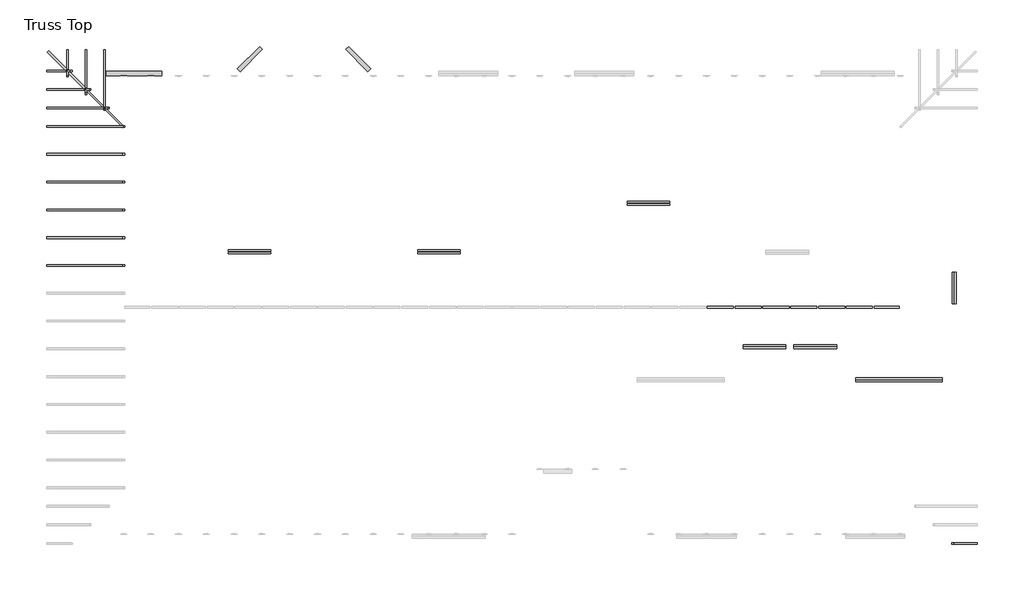
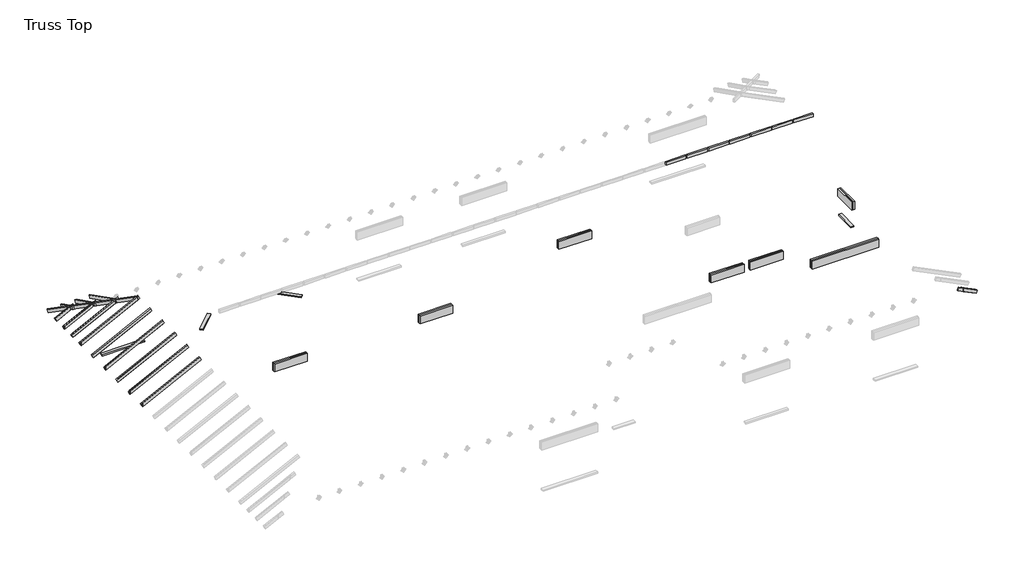
# One storey, part 2 of 3: 39 beams.
"""IFC4 building model written with IfcOpenShell, lengths in millimetres."""

import ifcopenshell
import ifcopenshell.guid

model = None  # the IFC model being written
_history = None  # IfcOwnerHistory: only IFC2X3 demands one
_inside = {}  # id of a spatial element -> (the spatial element, [elements in it])
_under = {}  # id of a project, library or spatial element -> (it, [spatial elements below it])
_declared = {}  # id of a project -> (the project, [libraries it declares])
_typed = {}  # id of a type object -> (the type object, [elements of that type])
_made_of = {}  # id of a material, layer set ... -> (it, [elements and type objects made of it])


def new_model(schema):
    """Start an empty IFC model of exactly this schema.

    Asked for "IFC4X3", IfcOpenShell would pick the latest addendum, in which some entities
    have other attributes; the version numbers below select the first issue.
    IFC2X3 requires an IfcOwnerHistory on every rooted entity: one is made here for all.
    """
    global model, _history
    if schema == "IFC4X3":
        model = ifcopenshell.file(schema_version=(4, 3, 0, 0))
    else:
        model = ifcopenshell.file(schema=schema)
    _inside.clear()
    _under.clear()
    _declared.clear()
    _typed.clear()
    _made_of.clear()
    _history = None
    if model.schema == "IFC2X3":
        org = make("IfcOrganization", Name="unknown")
        user = make(
            "IfcPersonAndOrganization",
            ThePerson=make("IfcPerson", FamilyName="unknown"),
            TheOrganization=org,
        )
        app = make(
            "IfcApplication",
            ApplicationDeveloper=org,
            Version="unknown",
            ApplicationFullName="unknown",
            ApplicationIdentifier="unknown",
        )
        _history = make(
            "IfcOwnerHistory",
            OwningUser=user,
            OwningApplication=app,
            ChangeAction="ADDED",
            CreationDate=0,
        )
    return model


def make(cls, **values):
    """One entity of the class cls with the attributes given. An attribute that is None is left unset."""
    return model.create_entity(
        cls, **{name: value for name, value in values.items() if value is not None}
    )


def rooted(cls, **values):
    """An entity with a GlobalId (a new one), such as an element, a storey or a relation."""
    return make(cls, GlobalId=ifcopenshell.guid.new(), OwnerHistory=_history, **values)


def si_unit(unit_type, name, prefix=None):
    """IfcSIUnit, for example si_unit("LENGTHUNIT", "METRE", prefix="MILLI")."""
    return make("IfcSIUnit", UnitType=unit_type, Prefix=prefix, Name=name)


def assignment(units):
    """IfcUnitAssignment: the units of a project."""
    return None if units is None else make("IfcUnitAssignment", Units=units)


def point(xyz):
    """IfcCartesianPoint."""
    return None if xyz is None else make("IfcCartesianPoint", Coordinates=xyz)


def direction(xyz):
    """IfcDirection."""
    return None if xyz is None else make("IfcDirection", DirectionRatios=xyz)


def frame(location, z_axis=None, x_axis=None):
    """IfcAxis2Placement3D, a coordinate frame: its origin and axes. An axis left out is left unset."""
    return make(
        "IfcAxis2Placement3D",
        Location=point(location),
        Axis=direction(z_axis),
        RefDirection=direction(x_axis),
    )


def origin():
    """The frame at (0, 0, 0) with its axes left unset."""
    return frame((0.0, 0.0, 0.0))


def place(relative_to, where):
    """IfcLocalPlacement: puts the frame where relative to a parent placement (None: the world)."""
    return make(
        "IfcLocalPlacement", PlacementRelTo=relative_to, RelativePlacement=where
    )


def context(
    kind, dimensions, precision=None, world=None, true_north=None, identifier=None
):
    """IfcGeometricRepresentationContext, for example the 3D "Model" context."""
    return make(
        "IfcGeometricRepresentationContext",
        ContextIdentifier=identifier,
        ContextType=kind,
        CoordinateSpaceDimension=dimensions,
        Precision=precision,
        WorldCoordinateSystem=world,
        TrueNorth=true_north,
    )


def project(units=None, contexts=None):
    """IfcProject with its units and contexts."""
    return rooted(
        "IfcProject",
        Name="project",
        RepresentationContexts=contexts,
        UnitsInContext=assignment(units),
    )


def spatial(cls, under=None, at=None, **own):
    """A site, building, storey or space (cls), placed at a placement, below another one or the project."""
    s = rooted(cls, ObjectPlacement=at, **own)
    if under is not None:
        _under.setdefault(under.id(), (under, []))[1].append(s)
    return s


def polyline(points):
    """IfcPolyline through the points."""
    return make("IfcPolyline", Points=[point(p) for p in points])


def outline(outer, holes=None, kind="AREA"):
    """IfcArbitraryClosedProfileDef: a profile drawn as a closed curve; with holes, ...WithVoids."""
    if holes is None:
        return make("IfcArbitraryClosedProfileDef", ProfileType=kind, OuterCurve=outer)
    return make(
        "IfcArbitraryProfileDefWithVoids",
        ProfileType=kind,
        OuterCurve=outer,
        InnerCurves=holes,
    )


def extrude(swept, where, along, depth):
    """IfcExtrudedAreaSolid: the profile swept, set in the frame where, extruded along a direction by depth."""
    return make(
        "IfcExtrudedAreaSolid",
        SweptArea=swept,
        Position=where,
        ExtrudedDirection=direction(along),
        Depth=depth,
    )


def faces_of(points, faces, orient=None, outer=None):
    """IfcFace entities. A face is a list of loops; a loop is a list of indices into points, from 0.

    orient and outer hold one flag for each loop. By default every Orientation is true, the
    first loop of a face is its IfcFaceOuterBound and the others are IfcFaceBound.
    """
    made = []
    for i, loops in enumerate(faces):
        bounds = []
        for j, loop in enumerate(loops):
            is_outer = j == 0 if outer is None else outer[i][j]
            bounds.append(
                make(
                    "IfcFaceOuterBound" if is_outer else "IfcFaceBound",
                    Bound=make("IfcPolyLoop", Polygon=[points[k] for k in loop]),
                    Orientation=True if orient is None else orient[i][j],
                )
            )
        made.append(make("IfcFace", Bounds=bounds))
    return made


def faceted_brep(points, faces, orient=None, outer=None, voids=None):
    """IfcFacetedBrep: a solid bounded by flat faces; with voids (closed shells), ...WithVoids."""
    shared = [point(p) for p in points]
    hull = make("IfcClosedShell", CfsFaces=faces_of(shared, faces, orient, outer))
    if voids is None:
        return make("IfcFacetedBrep", Outer=hull)
    return make(
        "IfcFacetedBrepWithVoids",
        Outer=hull,
        Voids=[
            make(cls, CfsFaces=faces_of(shared, fs, o, b)) for cls, fs, o, b in voids
        ],
    )


def shape(context_of_items, identifier, shape_type, items):
    """IfcShapeRepresentation: the items that make up one representation, for example the "Body"."""
    return make(
        "IfcShapeRepresentation",
        ContextOfItems=context_of_items,
        RepresentationIdentifier=identifier,
        RepresentationType=shape_type,
        Items=items,
    )


def source(mapping_origin, context_of_items, identifier, shape_type, items):
    """IfcRepresentationMap: a shape defined once, which mapped items show again and again."""
    return make(
        "IfcRepresentationMap",
        MappingOrigin=mapping_origin,
        MappedRepresentation=shape(context_of_items, identifier, shape_type, items),
    )


def transform(
    local_origin,
    x_axis=None,
    y_axis=None,
    z_axis=None,
    scale=None,
    scale2=None,
    scale3=None,
    uniform=True,
):
    """IfcCartesianTransformationOperator3D, or its non-uniform kind. x_axis, y_axis, z_axis: its Axis1, 2, 3."""
    if uniform:
        return make(
            "IfcCartesianTransformationOperator3D",
            Axis1=direction(x_axis),
            Axis2=direction(y_axis),
            LocalOrigin=point(local_origin),
            Scale=scale,
            Axis3=direction(z_axis),
        )
    return make(
        "IfcCartesianTransformationOperator3DnonUniform",
        Axis1=direction(x_axis),
        Axis2=direction(y_axis),
        LocalOrigin=point(local_origin),
        Scale=scale,
        Axis3=direction(z_axis),
        Scale2=scale2,
        Scale3=scale3,
    )


def mapped(mapping_source, mapping_target):
    """IfcMappedItem: shows the shape of a source again, moved by a transform."""
    return make(
        "IfcMappedItem", MappingSource=mapping_source, MappingTarget=mapping_target
    )


def made_of(thing, what):
    """Note that an element or type object is made of a material, layer set ...; save() writes the relation."""
    if what is not None:
        _made_of.setdefault(what.id(), (what, []))[1].append(thing)
    return thing


def element(
    cls,
    number,
    at=None,
    inside=None,
    cuts=None,
    type_object=None,
    material=None,
    context=None,
    identifier="Body",
    shape_type=None,
    held_by="IfcProductDefinitionShape",
    body=None,
    shapes=None,
    **own,
):
    """One element of the class cls, such as IfcWall. Its Tag is "e" and its number.

    at: its placement. inside: the storey or other place that contains it. cuts: it is an
    opening in that element (IfcRelVoidsElement). A single representation is given by context,
    identifier, shape_type and body (its items); several are given by shapes. held_by: the class
    of the entity that holds the representations. save() writes the other relations.
    """
    e = rooted(cls, Tag="e%d" % number, ObjectPlacement=at, **own)
    if body is not None:
        shapes = [shape(context, identifier, shape_type, body)]
    if shapes is not None:
        e.Representation = make(held_by, Representations=shapes)
    if inside is not None:
        _inside.setdefault(inside.id(), (inside, []))[1].append(e)
    if cuts is not None:
        rooted(
            "IfcRelVoidsElement", RelatingBuildingElement=cuts, RelatedOpeningElement=e
        )
    if type_object is not None:
        _typed.setdefault(type_object.id(), (type_object, []))[1].append(e)
    return made_of(e, material)


def aggregate(whole, parts):
    """IfcRelAggregates: a whole, such as a stair, and the parts it consists of."""
    return rooted("IfcRelAggregates", RelatingObject=whole, RelatedObjects=parts)


def save(model, path):
    """Write the relations noted so far, then the file.

    IfcRelAggregates (storeys below a building ...), IfcRelContainedInSpatialStructure (elements
    in a storey), IfcRelDefinesByType, IfcRelAssociatesMaterial and IfcRelDeclares: one each for
    every whole, place, type object, material and project.
    """
    for whole, parts in _under.values():
        aggregate(whole, parts)
    for where, things in _inside.values():
        rooted(
            "IfcRelContainedInSpatialStructure",
            RelatedElements=things,
            RelatingStructure=where,
        )
    for kind, things in _typed.values():
        rooted("IfcRelDefinesByType", RelatedObjects=things, RelatingType=kind)
    for what, things in _made_of.values():
        rooted("IfcRelAssociatesMaterial", RelatedObjects=things, RelatingMaterial=what)
    for by, libraries in _declared.values():
        rooted("IfcRelDeclares", RelatingContext=by, RelatedDefinitions=libraries)
    model.write(path)


def dimension_lumber_02b3d2e5(model_context):
    return source(origin(), model_context, "Body", "SweptSolid", [
        extrude(outline(polyline([(1211.111892, 19.05), (1211.111892, -19.05), (-1244.9189714, -19.05), (-1244.9189714, 19.05), (1211.111892, 19.05)])), frame((0.0, 0.0, -44.45), z_axis=(0.0, 0.0, 1.0), x_axis=(1.0, 0.0, 0.0)), (0.0, 0.0, 1.0), 88.9),
    ])


def dimension_lumber_26660400(model_context):
    return source(origin(), model_context, "Body", "SweptSolid", [
        extrude(outline(polyline([(276.225, 19.05), (276.225, -19.05), (-276.225, -19.05), (-276.225, 19.05), (276.225, 19.05)])), frame((0.0, 0.0, -44.45), z_axis=(0.0, 0.0, 1.0), x_axis=(1.0, 0.0, 0.0)), (0.0, 0.0, 1.0), 88.9),
    ])


def dimension_lumber_d546034e(model_context):
    return source(origin(), model_context, "Body", "SweptSolid", [
        extrude(outline(polyline([(295.275, 19.05), (295.275, -19.05), (-276.225, -19.05), (-276.225, 19.05), (295.275, 19.05)])), frame((0.0, 0.0, -44.45), z_axis=(0.0, 0.0, 1.0), x_axis=(1.0, 0.0, 0.0)), (0.0, 0.0, 1.0), 88.9),
    ])


def dimension_lumber_37c2d9e3(model_context):
    return source(origin(), model_context, "Body", "SweptSolid", [
        extrude(outline(polyline([(609.5999994, 44.45), (609.5999994, -44.45), (-609.5999994, -44.45), (-609.5999994, 44.45), (609.5999994, 44.45)])), frame((0.0, 0.0, -19.05), z_axis=(0.0, 0.0, 1.0), x_axis=(1.0, 0.0, 0.0)), (0.0, 0.0, 1.0), 38.1),
    ])


def dimension_lumber_e295fb9e(model_context):
    return source(origin(), model_context, "Body", "SweptSolid", [
        extrude(outline(polyline([(333.375, 44.45), (333.375, -44.45), (-352.4249994, -44.45), (-352.4249994, 44.45), (333.375, 44.45)])), frame((0.0, 0.0, -19.05), z_axis=(0.0, 0.0, 1.0), x_axis=(1.0, 0.0, 0.0)), (0.0, 0.0, 1.0), 38.1),
    ])


def dimension_lumber_05c0664a(model_context):
    return source(origin(), model_context, "Body", "SweptSolid", [
        extrude(outline(polyline([(333.375, -44.45), (-352.4249994, -44.45), (-352.4249994, 44.45), (333.375, 44.45), (333.375, -44.45)])), frame((0.0, 0.0, -19.05), z_axis=(0.0, 0.0, 1.0), x_axis=(1.0, 0.0, 0.0)), (0.0, 0.0, 1.0), 38.1),
    ])


def dimension_lumber_0879c48f(model_context):
    return source(origin(), model_context, "Body", "SweptSolid", [
        extrude(outline(polyline([(304.8, 44.45), (304.8, -44.45), (-304.8, -44.45), (-304.8, 44.45), (304.8, 44.45)])), frame((0.0, 0.0, -19.05), z_axis=(0.0, 0.0, 1.0), x_axis=(1.0, 0.0, 0.0)), (0.0, 0.0, 1.0), 38.1),
    ])


def dimension_lumber_2x10_header_exterior_80556d04(model_context):
    return source(origin(), model_context, "Body", "SweptSolid", [
        extrude(outline(polyline([(265.509375, 19.05), (265.509375, -19.05), (-420.290625, -19.05), (-420.290625, 19.05), (265.509375, 19.05)])), frame((0.0, 0.0, -117.475), z_axis=(0.0, 0.0, 1.0), x_axis=(1.0, 0.0, 0.0)), (0.0, 0.0, 1.0), 234.95),
    ])


def dimension_lumber_2x10_header_exterior_dd7e88d1(model_context):
    return source(origin(), model_context, "Body", "SweptSolid", [
        extrude(outline(polyline([(468.709375, 19.05), (468.709375, -19.05), (-468.709375, -19.05), (-468.709375, 19.05), (468.709375, 19.05)])), frame((0.0, 0.0, -117.475), z_axis=(0.0, 0.0, 1.0), x_axis=(1.0, 0.0, 0.0)), (0.0, 0.0, 1.0), 234.95),
    ])


def dimension_lumber_2x10_header_interior_e412fa49(model_context):
    return source(origin(), model_context, "Body", "SweptSolid", [
        extrude(outline(polyline([(468.709375, 19.05), (468.709375, -19.05), (-471.090625, -19.05), (-471.090625, 19.05), (468.709375, 19.05)])), frame((0.0, 0.0, -117.475), z_axis=(0.0, 0.0, 1.0), x_axis=(1.0, 0.0, 0.0)), (0.0, 0.0, 1.0), 234.95),
    ])


def dimension_lumber_2x10_header_interior_91014728(model_context):
    return source(origin(), model_context, "Body", "SweptSolid", [
        extrude(outline(polyline([(468.709375, 19.05), (468.709375, -19.05), (-1434.7031244, -19.05), (-1434.7031244, 19.05), (468.709375, 19.05)])), frame((0.0, 0.0, -117.475), z_axis=(0.0, 0.0, 1.0), x_axis=(1.0, 0.0, 0.0)), (0.0, 0.0, 1.0), 234.95),
    ])


model = new_model("IFC4")

# Units and contexts
model_context = context("Model", 3, world=origin())
ifc_project = project(units=[si_unit("LENGTHUNIT", "METRE", prefix="MILLI")], contexts=[model_context])

# Site, building, storey
site = spatial("IfcSite", under=ifc_project)
building = spatial("IfcBuilding", under=site)
storey = spatial("IfcBuildingStorey", under=building, Name="Truss Top", Elevation=5452.4432216)

# Beams
placement = place(None, origin())
element("IfcBeam", 1, ObjectType="Dimension Lumber : Roof Lumbers", at=placement, inside=storey, context=model_context, shape_type="SweptSolid", body=[
    extrude(outline(polyline([(0.0, -38.1), (0.0, 0.0), (1874.2721787, 0.0), (1874.2721787, -38.1), (0.0, -38.1)])), frame((-6669.4579365, 251.1959053, 2554.840297), z_axis=(-0.44721359549993395, 0.0, 0.894427190999928), x_axis=(0.894427190999928, 0.0, 0.44721359549993395)), (0.0, 0.0, 1.0), 88.9),
    extrude(outline(polyline([(2558.1548743, -6671.1152251), (2554.840297, -6669.4579365), (3393.040297, -4993.0579365), (3472.5548743, -5032.8152251), (2653.4048743, -6671.1152251), (2558.1548743, -6671.1152251)])), frame((0.0, 213.0959053, 0.0), z_axis=(0.0, 1.0, 0.0), x_axis=(0.0, 0.0, 1.0)), (0.0, 0.0, 1.0), 38.1),
    extrude(outline(polyline([(2564.60625, -6649.9260305), (3393.040297, -4993.0579365), (3472.5548743, -5032.8152251), (2653.4048743, -6671.1152251), (2564.60625, -6671.1152251), (2564.60625, -6649.9260305)])), frame((0.0, 213.0959053, 0.0), z_axis=(0.0, 1.0, 0.0), x_axis=(0.0, 0.0, 1.0)), (0.0, 0.0, 1.0), 38.1),
    extrude(outline(polyline([(2564.60625, -6649.9260305), (3373.1616527, -5032.8152251), (3472.5548743, -5032.8152251), (2653.4048743, -6671.1152251), (2564.60625, -6671.1152251), (2564.60625, -6649.9260305)])), frame((0.0, 213.0959053, 0.0), z_axis=(0.0, 1.0, 0.0), x_axis=(0.0, 0.0, 1.0)), (0.0, 0.0, 1.0), 38.1),
])
element("IfcBeam", 2, ObjectType="Dimension Lumber : Roof Lumbers", at=placement, inside=storey, context=model_context, shape_type="SweptSolid", body=[
    extrude(outline(polyline([(0.0, -38.1), (0.0, 0.0), (1874.2721787, 0.0), (1874.2721787, -38.1), (0.0, -38.1)])), frame((-6669.4579365, 860.7959053, 2554.840297), z_axis=(-0.44721359549993367, 0.0, 0.8944271909999281), x_axis=(0.8944271909999281, 0.0, 0.44721359549993367)), (0.0, 0.0, 1.0), 88.9),
    extrude(outline(polyline([(2558.1548743, -6671.1152251), (2554.840297, -6669.4579365), (3393.040297, -4993.0579365), (3472.5548743, -5032.8152251), (2653.4048743, -6671.1152251), (2558.1548743, -6671.1152251)])), frame((0.0, 822.6959053, 0.0), z_axis=(0.0, 1.0, 0.0), x_axis=(0.0, 0.0, 1.0)), (0.0, 0.0, 1.0), 38.1),
    extrude(outline(polyline([(2564.60625, -6649.9260305), (3393.040297, -4993.0579365), (3472.5548743, -5032.8152251), (2653.4048743, -6671.1152251), (2564.60625, -6671.1152251), (2564.60625, -6649.9260305)])), frame((0.0, 822.6959053, 0.0), z_axis=(0.0, 1.0, 0.0), x_axis=(0.0, 0.0, 1.0)), (0.0, 0.0, 1.0), 38.1),
    extrude(outline(polyline([(2564.60625, -6649.9260305), (3373.1616527, -5032.8152251), (3472.5548743, -5032.8152251), (2653.4048743, -6671.1152251), (2564.60625, -6671.1152251), (2564.60625, -6649.9260305)])), frame((0.0, 822.6959053, 0.0), z_axis=(0.0, 1.0, 0.0), x_axis=(0.0, 0.0, 1.0)), (0.0, 0.0, 1.0), 38.1),
])
element("IfcBeam", 3, ObjectType="Dimension Lumber : Roof Lumbers", at=placement, inside=storey, context=model_context, shape_type="SweptSolid", body=[
    extrude(outline(polyline([(0.0, -38.1), (0.0, 0.0), (1874.2721787, 0.0), (1874.2721787, -38.1), (0.0, -38.1)])), frame((-6669.4579365, 1470.3959053, 2554.840297), z_axis=(-0.44721359549993367, 0.0, 0.8944271909999281), x_axis=(0.8944271909999281, 0.0, 0.44721359549993367)), (0.0, 0.0, 1.0), 88.9),
    extrude(outline(polyline([(2558.1548743, -6671.1152251), (2554.840297, -6669.4579365), (3393.040297, -4993.0579365), (3472.5548743, -5032.8152251), (2653.4048743, -6671.1152251), (2558.1548743, -6671.1152251)])), frame((0.0, 1432.2959053, 0.0), z_axis=(0.0, 1.0, 0.0), x_axis=(0.0, 0.0, 1.0)), (0.0, 0.0, 1.0), 38.1),
    extrude(outline(polyline([(2564.60625, -6649.9260305), (3393.040297, -4993.0579365), (3472.5548743, -5032.8152251), (2653.4048743, -6671.1152251), (2564.60625, -6671.1152251), (2564.60625, -6649.9260305)])), frame((0.0, 1432.2959053, 0.0), z_axis=(0.0, 1.0, 0.0), x_axis=(0.0, 0.0, 1.0)), (0.0, 0.0, 1.0), 38.1),
    extrude(outline(polyline([(2564.60625, -6649.9260305), (3373.1616527, -5032.8152251), (3472.5548743, -5032.8152251), (2653.4048743, -6671.1152251), (2564.60625, -6671.1152251), (2564.60625, -6649.9260305)])), frame((0.0, 1432.2959053, 0.0), z_axis=(0.0, 1.0, 0.0), x_axis=(0.0, 0.0, 1.0)), (0.0, 0.0, 1.0), 38.1),
])
element("IfcBeam", 4, ObjectType="Dimension Lumber : Roof Lumbers", at=placement, inside=storey, context=model_context, shape_type="SweptSolid", body=[
    extrude(outline(polyline([(0.0, -38.1), (0.0, 0.0), (1874.2721787, 0.0), (1874.2721787, -38.1), (0.0, -38.1)])), frame((-6669.4579365, 2079.9959053, 2554.840297), z_axis=(-0.4472135954999335, 0.0, 0.8944271909999282), x_axis=(0.8944271909999282, 0.0, 0.4472135954999335)), (0.0, 0.0, 1.0), 88.9),
    extrude(outline(polyline([(2558.1548743, -6671.1152251), (2554.840297, -6669.4579365), (3393.040297, -4993.0579365), (3472.5548743, -5032.8152251), (2653.4048743, -6671.1152251), (2558.1548743, -6671.1152251)])), frame((0.0, 2041.8959053, 0.0), z_axis=(0.0, 1.0, 0.0), x_axis=(0.0, 0.0, 1.0)), (0.0, 0.0, 1.0), 38.1),
    extrude(outline(polyline([(2564.60625, -6649.9260305), (3393.040297, -4993.0579365), (3472.5548743, -5032.8152251), (2653.4048743, -6671.1152251), (2564.60625, -6671.1152251), (2564.60625, -6649.9260305)])), frame((0.0, 2041.8959053, 0.0), z_axis=(0.0, 1.0, 0.0), x_axis=(0.0, 0.0, 1.0)), (0.0, 0.0, 1.0), 38.1),
    extrude(outline(polyline([(2564.60625, -6649.9260305), (3373.1616527, -5032.8152251), (3472.5548743, -5032.8152251), (2653.4048743, -6671.1152251), (2564.60625, -6671.1152251), (2564.60625, -6649.9260305)])), frame((0.0, 2041.8959053, 0.0), z_axis=(0.0, 1.0, 0.0), x_axis=(0.0, 0.0, 1.0)), (0.0, 0.0, 1.0), 38.1),
])
element("IfcBeam", 5, ObjectType="Dimension Lumber : Roof Lumbers", at=placement, inside=storey, context=model_context, shape_type="SweptSolid", body=[
    extrude(outline(polyline([(0.0, -38.1), (0.0, 0.0), (1874.2721787, 0.0), (1874.2721787, -38.1), (0.0, -38.1)])), frame((-6669.4579365, 2689.5959053, 2554.840297), z_axis=(-0.4472135954999337, 0.0, 0.8944271909999281), x_axis=(0.8944271909999281, 0.0, 0.4472135954999337)), (0.0, 0.0, 1.0), 88.9),
    extrude(outline(polyline([(2558.1548743, -6671.1152251), (2554.840297, -6669.4579365), (3393.040297, -4993.0579365), (3472.5548743, -5032.8152251), (2653.4048743, -6671.1152251), (2558.1548743, -6671.1152251)])), frame((0.0, 2651.4959053, 0.0), z_axis=(0.0, 1.0, 0.0), x_axis=(0.0, 0.0, 1.0)), (0.0, 0.0, 1.0), 38.1),
    extrude(outline(polyline([(2564.60625, -6649.9260305), (3393.040297, -4993.0579365), (3472.5548743, -5032.8152251), (2653.4048743, -6671.1152251), (2564.60625, -6671.1152251), (2564.60625, -6649.9260305)])), frame((0.0, 2651.4959053, 0.0), z_axis=(0.0, 1.0, 0.0), x_axis=(0.0, 0.0, 1.0)), (0.0, 0.0, 1.0), 38.1),
    extrude(outline(polyline([(2564.60625, -6649.9260305), (3373.1616527, -5032.8152251), (3472.5548743, -5032.8152251), (2653.4048743, -6671.1152251), (2564.60625, -6671.1152251), (2564.60625, -6649.9260305)])), frame((0.0, 2651.4959053, 0.0), z_axis=(0.0, 1.0, 0.0), x_axis=(0.0, 0.0, 1.0)), (0.0, 0.0, 1.0), 38.1),
])
element("IfcBeam", 6, ObjectType="Dimension Lumber : Roof Lumbers", at=placement, inside=storey, context=model_context, shape_type="SweptSolid", body=[
    extrude(outline(polyline([(0.0, 38.1), (1877.0701871, 38.1), (1877.0701871, 0.0), (0.0, 0.0), (0.0, 38.1)])), frame((-6669.4579365, 3261.0959053, 2554.840297), z_axis=(-0.44721359549993367, 0.0, 0.8944271909999281), x_axis=(0.8944271909999281, 0.0, 0.44721359549993367)), (0.0, 0.0, 1.0), 88.9),
    extrude(outline(polyline([(2554.840297, -6669.4579365), (3394.2916044, -4990.5553218), (3473.8061816, -5030.3126104), (2653.4048743, -6671.1152251), (2558.1548743, -6671.1152251), (2554.840297, -6669.4579365)])), frame((0.0, 3261.0959053, 0.0), z_axis=(0.0, 1.0, 0.0), x_axis=(0.0, 0.0, 1.0)), (0.0, 0.0, 1.0), 38.1),
    extrude(outline(polyline([(2564.60625, -6649.9260305), (3394.2916044, -4990.5553218), (3473.8061816, -5030.3126104), (2653.4048743, -6671.1152251), (2564.60625, -6671.1152251), (2564.60625, -6649.9260305)])), frame((0.0, 3261.0959053, 0.0), z_axis=(0.0, 1.0, 0.0), x_axis=(0.0, 0.0, 1.0)), (0.0, 0.0, 1.0), 38.1),
    extrude(outline(polyline([(2564.60625, -6649.9260305), (3373.1616527, -5032.8152251), (3472.5548743, -5032.8152251), (2653.4048743, -6671.1152251), (2564.60625, -6671.1152251), (2564.60625, -6649.9260305)])), frame((0.0, 3261.0959053, 0.0), z_axis=(0.0, 1.0, 0.0), x_axis=(0.0, 0.0, 1.0)), (0.0, 0.0, 1.0), 38.1),
])
element("IfcBeam", 7, ObjectType="Dimension Lumber : Roof Lumbers", at=placement, inside=storey, context=model_context, shape_type="Brep", body=[
    faceted_brep([(13712.3847749, -5882.9040947, 2634.3548743), (13672.6274862, -5882.9040947, 2554.840297), (13672.6274862, -5844.8040947, 2554.840297), (13712.3847749, -5844.8040947, 2634.3548743), (13189.8604099, -5882.9040947, 2895.6170568), (13189.8604099, -5844.8040947, 2895.6170568), (13150.1031213, -5844.8040947, 2816.1024795), (13150.1031213, -5882.9040947, 2816.1024795)], [[[0, 1, 2, 3]], [[4, 5, 6, 7]], [[3, 5, 4, 0]], [[2, 6, 5, 3]], [[1, 7, 6, 2]], [[0, 4, 7, 1]]]),
    faceted_brep([(13712.3847749, -5882.9040947, 2634.3548743), (13672.6274862, -5882.9040947, 2554.840297), (13672.6274862, -5844.8040947, 2554.840297), (13712.3847749, -5844.8040947, 2634.3548743), (13301.1755432, -5882.9040947, 2839.9594901), (13301.1755432, -5882.9040947, 2740.5662685), (13263.0755432, -5844.8040947, 2759.6162685), (13263.0755432, -5844.8040947, 2859.0094901)], [[[0, 1, 2, 3]], [[0, 4, 5, 1]], [[1, 5, 6, 2]], [[2, 6, 7, 3]], [[3, 7, 4, 0]], [[4, 7, 6, 5]]]),
    faceted_brep([(13674.2847749, -5882.9040947, 2558.1548743), (13674.2847749, -5844.8040947, 2558.1548743), (13674.2847749, -5844.8040947, 2653.4048743), (13674.2847749, -5882.9040947, 2653.4048743), (13672.6274862, -5882.9040947, 2554.840297), (13672.6274862, -5844.8040947, 2554.840297), (13301.1755432, -5882.9040947, 2839.9594901), (13301.1755432, -5882.9040947, 2740.5662685), (13263.0755432, -5844.8040947, 2759.6162685), (13263.0755432, -5844.8040947, 2859.0094901)], [[[0, 1, 2, 3]], [[0, 4, 5, 1]], [[3, 6, 7, 4, 0]], [[4, 7, 8, 5]], [[5, 8, 9, 2, 1]], [[2, 9, 6, 3]], [[6, 9, 8, 7]]]),
])
element("IfcBeam", 8, ObjectType="Dimension Lumber : Roof Lumbers", at=placement, inside=storey, context=model_context, shape_type="Brep", body=[
    faceted_brep([(-5458.2652251, 3677.4390525, 3273.9083007), (-5458.2652251, 3637.6817638, 3194.3937234), (-5420.1652251, 3637.6817638, 3194.3937234), (-5420.1652251, 3677.4390525, 3273.9083007), (-5458.2652251, 4964.5299027, 2630.3628756), (-5420.1652251, 4964.5299027, 2630.3628756), (-5420.1652251, 4924.7726141, 2550.8482983), (-5458.2652251, 4924.7726141, 2550.8482983)], [[[0, 1, 2, 3]], [[4, 5, 6, 7]], [[3, 5, 4, 0]], [[2, 6, 5, 3]], [[1, 7, 6, 2]], [[0, 4, 7, 1]]]),
    faceted_brep([(-5458.2652251, 4964.5299027, 2630.3628756), (-5420.1652251, 4964.5299027, 2630.3628756), (-5420.1652251, 4924.7726141, 2550.8482983), (-5458.2652251, 4924.7726141, 2550.8482983), (-5420.1652251, 3694.4366737, 3265.4094901), (-5458.2652251, 3732.5366737, 3246.3594901), (-5420.1652251, 3694.4366737, 3166.0162685), (-5458.2652251, 3732.5366737, 3146.9662685)], [[[0, 1, 2, 3]], [[4, 1, 0, 5]], [[6, 2, 1, 4]], [[7, 3, 2, 6]], [[5, 0, 3, 7]], [[4, 5, 7, 6]]]),
    faceted_brep([(-5420.1652251, 3694.4366737, 3166.0162685), (-5420.1652251, 4918.4459053, 2554.0116527), (-5420.1652251, 4918.4459053, 2653.4048743), (-5420.1652251, 3694.4366737, 3265.4094901), (-5458.2652251, 4918.4459053, 2653.4048743), (-5458.2652251, 3732.5366737, 3246.3594901), (-5458.2652251, 4918.4459053, 2554.0116527), (-5458.2652251, 3732.5366737, 3146.9662685)], [[[0, 1, 2, 3]], [[3, 2, 4, 5]], [[5, 4, 6, 7]], [[3, 5, 7, 0]], [[7, 6, 1, 0]], [[4, 2, 1, 6]]]),
    faceted_brep([(-5458.2652251, 3732.5366737, 3146.9662685), (-5458.2652251, 4897.2567107, 2564.60625), (-5420.1652251, 4897.2567107, 2564.60625), (-5420.1652251, 3694.4366737, 3166.0162685), (-5420.1652251, 4918.4459053, 2564.60625), (-5420.1652251, 4918.4459053, 2653.4048743), (-5420.1652251, 3694.4366737, 3265.4094901), (-5458.2652251, 4918.4459053, 2653.4048743), (-5458.2652251, 4918.4459053, 2564.60625), (-5458.2652251, 3732.5366737, 3246.3594901)], [[[0, 1, 2, 3]], [[3, 2, 4, 5, 6]], [[7, 5, 4, 8]], [[6, 5, 7, 9]], [[6, 9, 0, 3]], [[9, 7, 8, 1, 0]], [[4, 2, 1, 8]]]),
])
element("IfcBeam", 9, ObjectType="Dimension Lumber : Roof Lumbers", at=placement, inside=storey, context=model_context, shape_type="Brep", body=[
    faceted_brep([(-5864.6652251, 4020.6444286, 3102.3056127), (-5864.6652251, 3980.88714, 3022.7910354), (-5826.5652251, 3980.88714, 3022.7910354), (-5826.5652251, 4020.6444286, 3102.3056127), (-5864.6652251, 4964.5299027, 2630.3628756), (-5826.5652251, 4964.5299027, 2630.3628756), (-5826.5652251, 4924.7726141, 2550.8482983), (-5864.6652251, 4924.7726141, 2550.8482983)], [[[0, 1, 2, 3]], [[4, 5, 6, 7]], [[3, 5, 4, 0]], [[2, 6, 5, 3]], [[1, 7, 6, 2]], [[0, 4, 7, 1]]]),
    faceted_brep([(-5864.6652251, 4964.5299027, 2630.3628756), (-5826.5652251, 4964.5299027, 2630.3628756), (-5826.5652251, 4924.7726141, 2550.8482983), (-5864.6652251, 4924.7726141, 2550.8482983), (-5826.5652251, 4100.8366737, 3062.2094901), (-5864.6652251, 4138.9366737, 3043.1594901), (-5826.5652251, 4100.8366737, 2962.8162685), (-5864.6652251, 4138.9366737, 2943.7662685)], [[[0, 1, 2, 3]], [[4, 1, 0, 5]], [[6, 2, 1, 4]], [[7, 3, 2, 6]], [[5, 0, 3, 7]], [[4, 5, 7, 6]]]),
    faceted_brep([(-5826.5652251, 4100.8366737, 2962.8162685), (-5826.5652251, 4918.4459053, 2554.0116527), (-5826.5652251, 4918.4459053, 2653.4048743), (-5826.5652251, 4100.8366737, 3062.2094901), (-5864.6652251, 4918.4459053, 2653.4048743), (-5864.6652251, 4138.9366737, 3043.1594901), (-5864.6652251, 4918.4459053, 2554.0116527), (-5864.6652251, 4138.9366737, 2943.7662685)], [[[0, 1, 2, 3]], [[3, 2, 4, 5]], [[5, 4, 6, 7]], [[3, 5, 7, 0]], [[7, 6, 1, 0]], [[4, 2, 1, 6]]]),
    faceted_brep([(-5864.6652251, 4138.9366737, 2943.7662685), (-5864.6652251, 4897.2567107, 2564.60625), (-5826.5652251, 4897.2567107, 2564.60625), (-5826.5652251, 4100.8366737, 2962.8162685), (-5826.5652251, 4918.4459053, 2564.60625), (-5826.5652251, 4918.4459053, 2653.4048743), (-5826.5652251, 4100.8366737, 3062.2094901), (-5864.6652251, 4918.4459053, 2653.4048743), (-5864.6652251, 4918.4459053, 2564.60625), (-5864.6652251, 4138.9366737, 3043.1594901)], [[[0, 1, 2, 3]], [[3, 2, 4, 5, 6]], [[7, 5, 4, 8]], [[6, 5, 7, 9]], [[6, 9, 0, 3]], [[9, 7, 8, 1, 0]], [[4, 2, 1, 8]]]),
])
element("IfcBeam", 10, ObjectType="Dimension Lumber : Roof Lumbers", at=placement, inside=storey, context=model_context, shape_type="Brep", body=[
    faceted_brep([(-6271.0652251, 4406.8580897, 2909.1987821), (-6271.0652251, 4367.100801, 2829.6842048), (-6232.9652251, 4367.100801, 2829.6842048), (-6232.9652251, 4406.8580897, 2909.1987821), (-6271.0652251, 4964.5299027, 2630.3628756), (-6232.9652251, 4964.5299027, 2630.3628756), (-6232.9652251, 4924.7726141, 2550.8482983), (-6271.0652251, 4924.7726141, 2550.8482983)], [[[0, 1, 2, 3]], [[4, 5, 6, 7]], [[3, 5, 4, 0]], [[2, 6, 5, 3]], [[1, 7, 6, 2]], [[0, 4, 7, 1]]]),
    faceted_brep([(-6271.0652251, 4964.5299027, 2630.3628756), (-6232.9652251, 4964.5299027, 2630.3628756), (-6232.9652251, 4924.7726141, 2550.8482983), (-6271.0652251, 4924.7726141, 2550.8482983), (-6232.9652251, 4507.2366737, 2859.0094901), (-6271.0652251, 4545.3366737, 2839.9594901), (-6232.9652251, 4507.2366737, 2759.6162685), (-6271.0652251, 4545.3366737, 2740.5662685)], [[[0, 1, 2, 3]], [[4, 1, 0, 5]], [[6, 2, 1, 4]], [[7, 3, 2, 6]], [[5, 0, 3, 7]], [[4, 5, 7, 6]]]),
    faceted_brep([(-6232.9652251, 4507.2366737, 2759.6162685), (-6232.9652251, 4918.4459053, 2554.0116527), (-6232.9652251, 4918.4459053, 2653.4048743), (-6232.9652251, 4507.2366737, 2859.0094901), (-6271.0652251, 4918.4459053, 2653.4048743), (-6271.0652251, 4545.3366737, 2839.9594901), (-6271.0652251, 4918.4459053, 2554.0116527), (-6271.0652251, 4545.3366737, 2740.5662685)], [[[0, 1, 2, 3]], [[3, 2, 4, 5]], [[5, 4, 6, 7]], [[3, 5, 7, 0]], [[7, 6, 1, 0]], [[4, 2, 1, 6]]]),
    faceted_brep([(-6271.0652251, 4545.3366737, 2740.5662685), (-6271.0652251, 4897.2567107, 2564.60625), (-6232.9652251, 4897.2567107, 2564.60625), (-6232.9652251, 4507.2366737, 2759.6162685), (-6232.9652251, 4918.4459053, 2564.60625), (-6232.9652251, 4918.4459053, 2653.4048743), (-6232.9652251, 4507.2366737, 2859.0094901), (-6271.0652251, 4918.4459053, 2653.4048743), (-6271.0652251, 4918.4459053, 2564.60625), (-6271.0652251, 4545.3366737, 2839.9594901)], [[[0, 1, 2, 3]], [[3, 2, 4, 5, 6]], [[7, 5, 4, 8]], [[6, 5, 7, 9]], [[6, 9, 0, 3]], [[9, 7, 8, 1, 0]], [[4, 2, 1, 8]]]),
])
element("IfcBeam", 11, ObjectType="Dimension Lumber : Roof Lumbers", at=placement, inside=storey, context=model_context, shape_type="Brep", body=[
    faceted_brep([(-6709.2152251, 3705.5959053, 2634.3548743), (-6669.4579365, 3705.5959053, 2554.840297), (-6669.4579365, 3667.4959053, 2554.840297), (-6709.2152251, 3667.4959053, 2634.3548743), (-5368.8266367, 3705.5959053, 3304.5491685), (-5368.8266367, 3667.4959053, 3304.5491685), (-5329.069348, 3667.4959053, 3225.0345912), (-5329.069348, 3705.5959053, 3225.0345912)], [[[0, 1, 2, 3]], [[4, 5, 6, 7]], [[3, 5, 4, 0]], [[2, 6, 5, 3]], [[1, 7, 6, 2]], [[0, 4, 7, 1]]]),
    faceted_brep([(-6709.2152251, 3705.5959053, 2634.3548743), (-6669.4579365, 3705.5959053, 2554.840297), (-6669.4579365, 3667.4959053, 2554.840297), (-6709.2152251, 3667.4959053, 2634.3548743), (-5485.2059935, 3705.5959053, 3246.3594901), (-5485.2059935, 3705.5959053, 3146.9662685), (-5447.1059935, 3667.4959053, 3166.0162685), (-5447.1059935, 3667.4959053, 3265.4094901)], [[[0, 1, 2, 3]], [[0, 4, 5, 1]], [[1, 5, 6, 2]], [[2, 6, 7, 3]], [[3, 7, 4, 0]], [[4, 7, 6, 5]]]),
    faceted_brep([(-6709.2152251, 3705.5959053, 2634.3548743), (-6674.340913, 3705.5959053, 2564.60625), (-6674.340913, 3667.4959053, 2564.60625), (-6709.2152251, 3667.4959053, 2634.3548743), (-5485.2059935, 3705.5959053, 3246.3594901), (-5485.2059935, 3705.5959053, 3146.9662685), (-6649.9260305, 3705.5959053, 2564.60625), (-6649.9260305, 3667.4959053, 2564.60625), (-5447.1059935, 3667.4959053, 3166.0162685), (-5447.1059935, 3667.4959053, 3265.4094901)], [[[0, 1, 2, 3]], [[0, 4, 5, 6, 1]], [[7, 8, 9, 3, 2]], [[3, 9, 4, 0]], [[4, 9, 8, 5]], [[6, 5, 8, 7]], [[2, 1, 6, 7]]]),
    faceted_brep([(-6671.1152251, 3667.4959053, 2653.4048743), (-5447.1059935, 3667.4959053, 3265.4094901), (-5485.2059935, 3705.5959053, 3246.3594901), (-6671.1152251, 3705.5959053, 2653.4048743), (-5485.2059935, 3705.5959053, 3146.9662685), (-6649.9260305, 3705.5959053, 2564.60625), (-6671.1152251, 3705.5959053, 2564.60625), (-5447.1059935, 3667.4959053, 3166.0162685), (-6649.9260305, 3667.4959053, 2564.60625), (-6671.1152251, 3667.4959053, 2564.60625)], [[[0, 1, 2, 3]], [[3, 2, 4, 5, 6]], [[2, 1, 7, 4]], [[5, 4, 7, 8]], [[6, 5, 8, 9]], [[8, 7, 1, 0, 9]], [[3, 6, 9, 0]]]),
])
element("IfcBeam", 12, ObjectType="Dimension Lumber : Roof Lumbers", at=placement, inside=storey, context=model_context, shape_type="Brep", body=[
    faceted_brep([(-6709.2152251, 4111.9959053, 2634.3548743), (-6669.4579365, 4111.9959053, 2554.840297), (-6669.4579365, 4073.8959053, 2554.840297), (-6709.2152251, 4073.8959053, 2634.3548743), (-5777.7587484, 4111.9959053, 3100.0831127), (-5777.7587484, 4073.8959053, 3100.0831127), (-5738.0014598, 4073.8959053, 3020.5685354), (-5738.0014598, 4111.9959053, 3020.5685354)], [[[0, 1, 2, 3]], [[4, 5, 6, 7]], [[3, 5, 4, 0]], [[2, 6, 5, 3]], [[1, 7, 6, 2]], [[0, 4, 7, 1]]]),
    faceted_brep([(-6709.2152251, 4111.9959053, 2634.3548743), (-6669.4579365, 4111.9959053, 2554.840297), (-6669.4579365, 4073.8959053, 2554.840297), (-6709.2152251, 4073.8959053, 2634.3548743), (-5891.6059935, 4111.9959053, 3043.1594901), (-5891.6059935, 4111.9959053, 2943.7662685), (-5853.5059935, 4073.8959053, 2962.8162685), (-5853.5059935, 4073.8959053, 3062.2094901)], [[[0, 1, 2, 3]], [[0, 4, 5, 1]], [[1, 5, 6, 2]], [[2, 6, 7, 3]], [[3, 7, 4, 0]], [[4, 7, 6, 5]]]),
    faceted_brep([(-6709.2152251, 4111.9959053, 2634.3548743), (-6674.340913, 4111.9959053, 2564.60625), (-6674.340913, 4073.8959053, 2564.60625), (-6709.2152251, 4073.8959053, 2634.3548743), (-5891.6059935, 4111.9959053, 3043.1594901), (-5891.6059935, 4111.9959053, 2943.7662685), (-6649.9260305, 4111.9959053, 2564.60625), (-6649.9260305, 4073.8959053, 2564.60625), (-5853.5059935, 4073.8959053, 2962.8162685), (-5853.5059935, 4073.8959053, 3062.2094901)], [[[0, 1, 2, 3]], [[0, 4, 5, 6, 1]], [[7, 8, 9, 3, 2]], [[3, 9, 4, 0]], [[4, 9, 8, 5]], [[6, 5, 8, 7]], [[2, 1, 6, 7]]]),
    faceted_brep([(-6671.1152251, 4073.8959053, 2653.4048743), (-5853.5059935, 4073.8959053, 3062.2094901), (-5891.6059935, 4111.9959053, 3043.1594901), (-6671.1152251, 4111.9959053, 2653.4048743), (-5891.6059935, 4111.9959053, 2943.7662685), (-6649.9260305, 4111.9959053, 2564.60625), (-6671.1152251, 4111.9959053, 2564.60625), (-5853.5059935, 4073.8959053, 2962.8162685), (-6649.9260305, 4073.8959053, 2564.60625), (-6671.1152251, 4073.8959053, 2564.60625)], [[[0, 1, 2, 3]], [[3, 2, 4, 5, 6]], [[2, 1, 7, 4]], [[5, 4, 7, 8]], [[6, 5, 8, 9]], [[8, 7, 1, 0, 9]], [[3, 6, 9, 0]]]),
])
element("IfcBeam", 13, ObjectType="Dimension Lumber : Roof Lumbers", at=placement, inside=storey, context=model_context, shape_type="Brep", body=[
    faceted_brep([(-6709.2152251, 4518.3959053, 2634.3548743), (-6669.4579365, 4518.3959053, 2554.840297), (-6669.4579365, 4480.2959053, 2554.840297), (-6709.2152251, 4480.2959053, 2634.3548743), (-6186.6908601, 4518.3959053, 2895.6170568), (-6186.6908601, 4480.2959053, 2895.6170568), (-6146.9335715, 4480.2959053, 2816.1024795), (-6146.9335715, 4518.3959053, 2816.1024795)], [[[0, 1, 2, 3]], [[4, 5, 6, 7]], [[3, 5, 4, 0]], [[2, 6, 5, 3]], [[1, 7, 6, 2]], [[0, 4, 7, 1]]]),
    faceted_brep([(-6709.2152251, 4518.3959053, 2634.3548743), (-6669.4579365, 4518.3959053, 2554.840297), (-6669.4579365, 4480.2959053, 2554.840297), (-6709.2152251, 4480.2959053, 2634.3548743), (-6298.0059935, 4518.3959053, 2839.9594901), (-6298.0059935, 4518.3959053, 2740.5662685), (-6259.9059935, 4480.2959053, 2759.6162685), (-6259.9059935, 4480.2959053, 2859.0094901)], [[[0, 1, 2, 3]], [[0, 4, 5, 1]], [[1, 5, 6, 2]], [[2, 6, 7, 3]], [[3, 7, 4, 0]], [[4, 7, 6, 5]]]),
    faceted_brep([(-6709.2152251, 4518.3959053, 2634.3548743), (-6674.340913, 4518.3959053, 2564.60625), (-6674.340913, 4480.2959053, 2564.60625), (-6709.2152251, 4480.2959053, 2634.3548743), (-6298.0059935, 4518.3959053, 2839.9594901), (-6298.0059935, 4518.3959053, 2740.5662685), (-6649.9260305, 4518.3959053, 2564.60625), (-6649.9260305, 4480.2959053, 2564.60625), (-6259.9059935, 4480.2959053, 2759.6162685), (-6259.9059935, 4480.2959053, 2859.0094901)], [[[0, 1, 2, 3]], [[0, 4, 5, 6, 1]], [[7, 8, 9, 3, 2]], [[3, 9, 4, 0]], [[4, 9, 8, 5]], [[6, 5, 8, 7]], [[2, 1, 6, 7]]]),
    faceted_brep([(-6671.1152251, 4480.2959053, 2653.4048743), (-6259.9059935, 4480.2959053, 2859.0094901), (-6298.0059935, 4518.3959053, 2839.9594901), (-6671.1152251, 4518.3959053, 2653.4048743), (-6298.0059935, 4518.3959053, 2740.5662685), (-6649.9260305, 4518.3959053, 2564.60625), (-6671.1152251, 4518.3959053, 2564.60625), (-6259.9059935, 4480.2959053, 2759.6162685), (-6649.9260305, 4480.2959053, 2564.60625), (-6671.1152251, 4480.2959053, 2564.60625)], [[[0, 1, 2, 3]], [[3, 2, 4, 5, 6]], [[2, 1, 7, 4]], [[5, 4, 7, 8]], [[6, 5, 8, 9]], [[8, 7, 1, 0, 9]], [[3, 6, 9, 0]]]),
])
dimension_lumber_shape = dimension_lumber_02b3d2e5(model_context)
element("IfcBeam", 14, ObjectType="Dimension Lumber : Roof Lumbers", at=placement, inside=storey, context=model_context, shape_type="MappedRepresentation", body=[
    mapped(dimension_lumber_shape, transform((-5859.0415503, 4106.3722305, 3005.560175), x_axis=(-0.6666666666666615, 0.6666666666666727, -0.3333333333333318), y_axis=(-0.7071067811865536, -0.7071067811865417, 0.0), z_axis=(-0.23570226039551276, 0.23570226039551673, 0.9428090415820639))),
])
dimension_lumber_2_shape = dimension_lumber_26660400(model_context)
element("IfcBeam", 15, ObjectType="Dimension Lumber : Roof Lumbers", at=placement, inside=storey, context=model_context, shape_type="MappedRepresentation", body=[
    mapped(dimension_lumber_2_shape, transform((11721.6597749, -682.2540947, 5399.6588466), x_axis=(-1.0, 0.0, 0.0), y_axis=(0.0, -1.0, 0.0), z_axis=(0.0, 0.0, 1.0))),
])
dimension_lumber_3_shape = dimension_lumber_d546034e(model_context)
element("IfcBeam", 16, ObjectType="Dimension Lumber : Roof Lumbers", at=placement, inside=storey, context=model_context, shape_type="MappedRepresentation", body=[
    mapped(dimension_lumber_3_shape, transform((11131.1097749, -682.2540947, 5399.6588466), x_axis=(-1.0, 0.0, 0.0), y_axis=(0.0, -1.0, 0.0), z_axis=(0.0, 0.0, 1.0))),
])
element("IfcBeam", 17, ObjectType="Dimension Lumber : Roof Lumbers", at=placement, inside=storey, context=model_context, shape_type="MappedRepresentation", body=[
    mapped(dimension_lumber_3_shape, transform((10521.5097749, -682.2540947, 5399.6588466), x_axis=(-1.0, 0.0, 0.0), y_axis=(0.0, -1.0, 0.0), z_axis=(0.0, 0.0, 1.0))),
])
element("IfcBeam", 18, ObjectType="Dimension Lumber : Roof Lumbers", at=placement, inside=storey, context=model_context, shape_type="MappedRepresentation", body=[
    mapped(dimension_lumber_3_shape, transform((9911.9097749, -682.2540947, 5399.6588466), x_axis=(-1.0, 0.0, 0.0), y_axis=(0.0, -1.0, 0.0), z_axis=(0.0, 0.0, 1.0))),
])
element("IfcBeam", 19, ObjectType="Dimension Lumber : Roof Lumbers", at=placement, inside=storey, context=model_context, shape_type="MappedRepresentation", body=[
    mapped(dimension_lumber_3_shape, transform((9302.3097749, -682.2540947, 5399.6588466), x_axis=(-1.0, 0.0, 0.0), y_axis=(0.0, -1.0, 0.0), z_axis=(0.0, 0.0, 1.0))),
])
element("IfcBeam", 20, ObjectType="Dimension Lumber : Roof Lumbers", at=placement, inside=storey, context=model_context, shape_type="MappedRepresentation", body=[
    mapped(dimension_lumber_3_shape, transform((8692.7097749, -682.2540947, 5399.6588466), x_axis=(-1.0, 0.0, 0.0), y_axis=(0.0, -1.0, 0.0), z_axis=(0.0, 0.0, 1.0))),
])
element("IfcBeam", 21, ObjectType="Dimension Lumber : Roof Lumbers", at=placement, inside=storey, context=model_context, shape_type="MappedRepresentation", body=[
    mapped(dimension_lumber_3_shape, transform((8083.1097749, -682.2540947, 5399.6588466), x_axis=(-1.0, 0.0, 0.0), y_axis=(0.0, -1.0, 0.0), z_axis=(0.0, 0.0, 1.0))),
])
dimension_lumber_4_shape = dimension_lumber_37c2d9e3(model_context)
element("IfcBeam", 22, ObjectType="Dimension Lumber : Opening Plate 2*4 Exterior", at=placement, inside=storey, context=model_context, shape_type="MappedRepresentation", body=[
    mapped(dimension_lumber_4_shape, transform((-4793.1027257, 4443.7834053, 1122.759375), x_axis=(1.0, 0.0, 0.0), y_axis=(0.0, 1.0, 0.0), z_axis=(0.0, 0.0, 1.0))),
])
dimension_lumber_5_shape = dimension_lumber_e295fb9e(model_context)
element("IfcBeam", 23, ObjectType="Dimension Lumber : Opening Plate 2*4 Exterior", at=placement, inside=storey, context=model_context, shape_type="MappedRepresentation", body=[
    mapped(dimension_lumber_5_shape, transform((-2240.3366366, 4768.337701, 817.959375), x_axis=(0.7071067811865549, 0.7071067811865402, 0.0), y_axis=(-0.7071067811865402, 0.7071067811865549, 0.0), z_axis=(0.0, 0.0, 1.0))),
])
dimension_lumber_6_shape = dimension_lumber_05c0664a(model_context)
element("IfcBeam", 24, ObjectType="Dimension Lumber : Opening Plate 2*4 Exterior", at=placement, inside=storey, context=model_context, shape_type="MappedRepresentation", body=[
    mapped(dimension_lumber_6_shape, transform((121.7311864, 4768.337701, 817.959375), x_axis=(-0.7071067811865549, 0.7071067811865402, 0.0), y_axis=(-0.7071067811865402, -0.7071067811865549, 0.0), z_axis=(0.0, 0.0, 1.0))),
])
dimension_lumber_7_shape = dimension_lumber_0879c48f(model_context)
element("IfcBeam", 25, ObjectType="Dimension Lumber : Opening Plate 2*4 Exterior", at=placement, inside=storey, context=model_context, shape_type="MappedRepresentation", body=[
    mapped(dimension_lumber_7_shape, transform((13199.6222749, -263.1540947, 1519.634375), x_axis=(0.0, -1.0, 0.0), y_axis=(1.0, 0.0, 0.0), z_axis=(0.0, 0.0, 1.0))),
])
dimension_lumber_2x10_header_exterior_shape = dimension_lumber_2x10_header_exterior_80556d04(model_context)
element("IfcBeam", 26, ObjectType="Dimension Lumber : 2x10 Header Exterior", at=placement, inside=storey, context=model_context, shape_type="MappedRepresentation", body=[
    mapped(dimension_lumber_2x10_header_exterior_shape, transform((13174.2222749, -185.7634697, 2173.684375), x_axis=(0.0, 1.0, 0.0), y_axis=(-1.0, 0.0, 0.0), z_axis=(0.0, 0.0, 1.0))),
])
element("IfcBeam", 27, ObjectType="Dimension Lumber : 2x10 Header Exterior", at=placement, inside=storey, context=model_context, shape_type="MappedRepresentation", body=[
    mapped(dimension_lumber_2x10_header_exterior_shape, transform((13225.0222749, -185.7634697, 2173.684375), x_axis=(0.0, 1.0, 0.0), y_axis=(-1.0, 0.0, 0.0), z_axis=(0.0, 0.0, 1.0))),
])
dimension_lumber_2x10_header_exterior_2_shape = dimension_lumber_2x10_header_exterior_dd7e88d1(model_context)
element("IfcBeam", 28, ObjectType="Dimension Lumber : 2x10 Header Interior", at=placement, inside=storey, context=model_context, shape_type="MappedRepresentation", body=[
    mapped(dimension_lumber_2x10_header_exterior_2_shape, transform((9038.7847749, -1571.2540947, 2173.684375), x_axis=(-1.0, 0.0, 0.0), y_axis=(0.0, -1.0, 0.0), z_axis=(0.0, 0.0, 1.0))),
])
element("IfcBeam", 29, ObjectType="Dimension Lumber : 2x10 Header Interior", at=placement, inside=storey, context=model_context, shape_type="MappedRepresentation", body=[
    mapped(dimension_lumber_2x10_header_exterior_2_shape, transform((9038.7847749, -1520.4540947, 2173.684375), x_axis=(-1.0, 0.0, 0.0), y_axis=(0.0, -1.0, 0.0), z_axis=(0.0, 0.0, 1.0))),
])
element("IfcBeam", 30, ObjectType="Dimension Lumber : 2x10 Header Interior", at=placement, inside=storey, context=model_context, shape_type="MappedRepresentation", body=[
    mapped(dimension_lumber_2x10_header_exterior_2_shape, transform((10156.3847749, -1571.2540947, 2173.684375), x_axis=(-1.0, 0.0, 0.0), y_axis=(0.0, -1.0, 0.0), z_axis=(0.0, 0.0, 1.0))),
])
element("IfcBeam", 31, ObjectType="Dimension Lumber : 2x10 Header Interior", at=placement, inside=storey, context=model_context, shape_type="MappedRepresentation", body=[
    mapped(dimension_lumber_2x10_header_exterior_2_shape, transform((10156.3847749, -1520.4540947, 2173.684375), x_axis=(-1.0, 0.0, 0.0), y_axis=(0.0, -1.0, 0.0), z_axis=(0.0, 0.0, 1.0))),
])
element("IfcBeam", 32, ObjectType="Dimension Lumber : 2x10 Header Interior", at=placement, inside=storey, context=model_context, shape_type="MappedRepresentation", body=[
    mapped(dimension_lumber_2x10_header_exterior_2_shape, transform((6493.6253999, 1571.9959053, 2173.684375), x_axis=(-1.0, 0.0, 0.0), y_axis=(0.0, -1.0, 0.0), z_axis=(0.0, 0.0, 1.0))),
])
element("IfcBeam", 33, ObjectType="Dimension Lumber : 2x10 Header Interior", at=placement, inside=storey, context=model_context, shape_type="MappedRepresentation", body=[
    mapped(dimension_lumber_2x10_header_exterior_2_shape, transform((6493.6253999, 1622.7959053, 2173.684375), x_axis=(-1.0, 0.0, 0.0), y_axis=(0.0, -1.0, 0.0), z_axis=(0.0, 0.0, 1.0))),
])
element("IfcBeam", 34, ObjectType="Dimension Lumber : 2x10 Header Interior", at=placement, inside=storey, context=model_context, shape_type="MappedRepresentation", body=[
    mapped(dimension_lumber_2x10_header_exterior_2_shape, transform((1901.3847749, 508.3709053, 2173.684375), x_axis=(-1.0, 0.0, 0.0), y_axis=(0.0, -1.0, 0.0), z_axis=(0.0, 0.0, 1.0))),
])
element("IfcBeam", 35, ObjectType="Dimension Lumber : 2x10 Header Interior", at=placement, inside=storey, context=model_context, shape_type="MappedRepresentation", body=[
    mapped(dimension_lumber_2x10_header_exterior_2_shape, transform((1901.3847749, 559.1709053, 2173.684375), x_axis=(-1.0, 0.0, 0.0), y_axis=(0.0, -1.0, 0.0), z_axis=(0.0, 0.0, 1.0))),
])
dimension_lumber_2x10_header_interior_shape = dimension_lumber_2x10_header_interior_e412fa49(model_context)
element("IfcBeam", 36, ObjectType="Dimension Lumber : 2x10 Header Interior", at=placement, inside=storey, context=model_context, shape_type="MappedRepresentation", body=[
    mapped(dimension_lumber_2x10_header_interior_shape, transform((-2259.8496001, 508.3709053, 2173.684375), x_axis=(-1.0, 0.0, 0.0), y_axis=(0.0, -1.0, 0.0), z_axis=(0.0, 0.0, 1.0))),
])
element("IfcBeam", 37, ObjectType="Dimension Lumber : 2x10 Header Interior", at=placement, inside=storey, context=model_context, shape_type="MappedRepresentation", body=[
    mapped(dimension_lumber_2x10_header_interior_shape, transform((-2259.8496001, 559.1709053, 2173.684375), x_axis=(-1.0, 0.0, 0.0), y_axis=(0.0, -1.0, 0.0), z_axis=(0.0, 0.0, 1.0))),
])
dimension_lumber_2x10_header_interior_2_shape = dimension_lumber_2x10_header_interior_91014728(model_context)
element("IfcBeam", 38, ObjectType="Dimension Lumber : 2x10 Header Interior", at=placement, inside=storey, context=model_context, shape_type="MappedRepresentation", body=[
    mapped(dimension_lumber_2x10_header_interior_2_shape, transform((11509.3316499, -2301.5040947, 2173.684375), x_axis=(-1.0, 0.0, 0.0), y_axis=(0.0, -1.0, 0.0), z_axis=(0.0, 0.0, 1.0))),
])
element("IfcBeam", 39, ObjectType="Dimension Lumber : 2x10 Header Interior", at=placement, inside=storey, context=model_context, shape_type="MappedRepresentation", body=[
    mapped(dimension_lumber_2x10_header_interior_2_shape, transform((11509.3316499, -2250.7040947, 2173.684375), x_axis=(-1.0, 0.0, 0.0), y_axis=(0.0, -1.0, 0.0), z_axis=(0.0, 0.0, 1.0))),
])

save(model, "model.ifc")

# Revit data of these elements
# Type "Dimension Lumber : Roof Lumbers"
#   Assembly Code = "B10"
#   A = 0.0364583 SF
#   Length [instance default] = 5' - 0"
#   b = 0' - 1 1/2"
#   d = 0' - 3 1/2"
#   Structural Material [instance default] = Softwood, Lumber
# Type "Dimension Lumber : Opening Plate 2*4 Exterior"
#   Assembly Code = "B10"
#   A = 0.0364583 SF
#   Length [instance default] = 5' - 0"
#   b = 0' - 3 1/2"
#   d = 0' - 1 1/2"
#   Structural Material [instance default] = Softwood, Lumber
# Type "Dimension Lumber : 2x10 Header Exterior"
#   Assembly Code = "B10"
#   A = 0.0963889 SF
#   Length [instance default] = 5' - 0"
#   b = 0' - 1 1/2"
#   d = 0' - 9 1/4"
#   Structural Material [instance default] = Softwood, Lumber
# Type "Dimension Lumber : 2x10 Header Interior"
#   Assembly Code = "B10"
#   A = 0.0963889 SF
#   Length [instance default] = 5' - 0"
#   b = 0' - 1 1/2"
#   d = 0' - 9 1/4"
#   Structural Material [instance default] = Softwood, Lumber
# Elements 1, 2, 3, 4, 5, 14, 15, 16, 17, 18, 19, 20, 21 (IfcBeam, "Dimension Lumber : Roof Lumbers")
#   Structural Material = Douglas Fir #2
#   Phase Created = New Construction
#   Materials on its faces: "Douglas Fir #2"
# Elements 6, 7, 8, 9, 10, 11, 12, 13 (IfcBeam, "Dimension Lumber : Roof Lumbers")
#   Structural Material = Softwood, Lumber
#   Phase Created = New Construction
#   Materials on its faces: "Softwood, Lumber"
# Elements 22, 23, 24, 25 (IfcBeam, "Dimension Lumber : Opening Plate 2*4 Exterior")
#   Structural Material = Douglas Fir #2
#   Phase Created = New Construction
#   Materials on its faces: "Douglas Fir #2"
# Elements 26, 27 (IfcBeam, "Dimension Lumber : 2x10 Header Exterior")
#   Comments = ""
#   Structural Material = Douglas Fir #2
#   Phase Created = New Construction
#   Materials on its faces: "Douglas Fir #2"
# Elements 28, 29, 30, 31, 32, 33, 34, 35, 36, 37, 38, 39 (IfcBeam, "Dimension Lumber : 2x10 Header Interior")
#   Comments = ""
#   Structural Material = Douglas Fir #2
#   Phase Created = New Construction
#   Materials on its faces: "Douglas Fir #2"
# Materials
#   "Softwood, Lumber": class "Wood", colour RGB 223 192 134, transparency 0, Description = "Pinus Echinata", Cost = 0
#   "Douglas Fir #2": class "Wood", colour RGB 223 192 134, transparency 0, Description = "Pinus Echinata", Cost = 0
